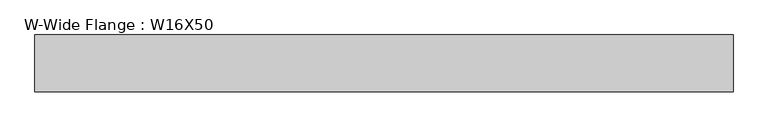
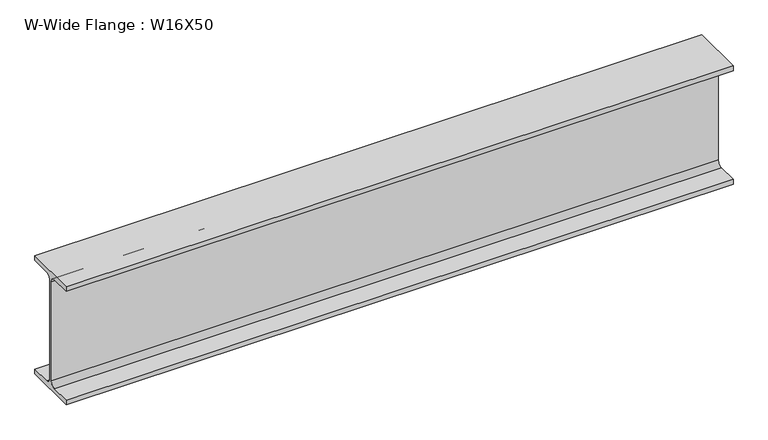
"""IFC4 building model written with IfcOpenShell, lengths in millimetres: beam geometry, W-Wide Flange : W16X50."""

from ifc_helpers import new_model, si_unit, point, frame, frame_2d, origin, place, context, project, spatial, polyline, circle_curve, trimmed, segment, composite_curve, outline, extrude, source, transform, mapped, element, save


def w_wide_flange_w16x50_2f8f61bc(model_context):
    return source(origin(), model_context, "Body", "SweptSolid", [
        extrude(outline(composite_curve([segment(polyline([(89.789, -191.008), (89.789, -207.01), (-89.789, -207.01), (-89.789, -191.008), (-22.1615, -191.008)]), True, "CONTINUOUS"), segment(trimmed(circle_curve(frame_2d((-22.1615, -173.6725)), 17.3355), [point((-22.1615, -191.008))], [point((-4.826, -173.6725))], True, "CARTESIAN"), True, "CONTINUOUS"), segment(polyline([(-4.826, -173.6725), (-4.826, 173.6725)]), True, "CONTINUOUS"), segment(trimmed(circle_curve(frame_2d((-22.1615, 173.6725)), 17.3355), [point((-4.826, 173.6725))], [point((-22.1615, 191.008))], True, "CARTESIAN"), True, "CONTINUOUS"), segment(polyline([(-22.1615, 191.008), (-89.789, 191.008), (-89.789, 207.01), (89.789, 207.01), (89.789, 191.008), (22.1615, 191.008)]), True, "CONTINUOUS"), segment(trimmed(circle_curve(frame_2d((22.1615, 173.6725)), 17.3355), [point((22.1615, 191.008))], [point((4.826, 173.6725))], True, "CARTESIAN"), True, "CONTINUOUS"), segment(polyline([(4.826, 173.6725), (4.826, -173.6725)]), True, "CONTINUOUS"), segment(trimmed(circle_curve(frame_2d((22.1615, -173.6725)), 17.3355), [point((4.826, -173.6725))], [point((22.1615, -191.008))], True, "CARTESIAN"), True, "CONTINUOUS"), segment(polyline([(22.1615, -191.008), (89.789, -191.008)]), True, "CONTINUOUS")], self_intersect=False)), frame((-1094.5030758, 0.0, 0.0), z_axis=(1.0, 0.0, 0.0), x_axis=(0.0, 1.0, 0.0)), (0.0, 0.0, 1.0), 2211.8661516),
    ])


if __name__ == "__main__":
    model = new_model("IFC4")
    model_context = context("Model", 3, world=origin())
    ifc_project = project(units=[si_unit("LENGTHUNIT", "METRE", prefix="MILLI")], contexts=[model_context])
    site = spatial("IfcSite", under=ifc_project)
    building = spatial("IfcBuilding", under=site)
    placement = place(None, origin())
    w_wide_flange_w16x50_shape = w_wide_flange_w16x50_2f8f61bc(model_context)
    element("IfcBeam", 1, ObjectType="W-Wide Flange : W16X50", at=placement, inside=building, context=model_context, shape_type="MappedRepresentation", body=[
        mapped(w_wide_flange_w16x50_shape, transform((0.0, 0.0, 0.0), x_axis=(1.0, 0.0, 0.0), y_axis=(0.0, 1.0, 0.0), z_axis=(0.0, 0.0, 1.0))),
    ])
    save(model, "model.ifc")

# Revit data of these elements
# Type "W-Wide Flange : W16X50"
#   Assembly Code = "B10"
#   W = 50
#   Start Extension Calculation [instance default] = 10' - 0"
#   Start Extension [instance default] = -0' - 0 1/2"
#   End Extension Calculation [instance default] = 10' - 0"
#   End Extension [instance default] = -0' - 0 1/2"
#   Length [instance default] = 5' - 0"
#   bf = 0' - 7.07"
#   d = 1' - 4.3"
#   k = 0' - 1 5/16"
#   k2 = 0' - 0.6825"
#   tf = 0' - 0.63"
#   tw = 0' - 0.38"
#   A = 0.102083 SF
#   Beam Material [instance default] = Metal - Steel - ASTM A992
# Element 1 (IfcBeam, "W-Wide Flange : W16X50")
#   Materials on its faces: "Metal - Steel - ASTM A992"
# Materials
#   "Metal - Steel - ASTM A992": class "Metal", colour RGB 128 0 0, transparency 0
